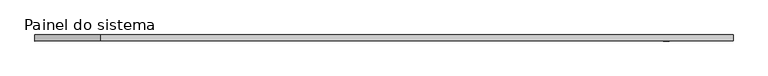
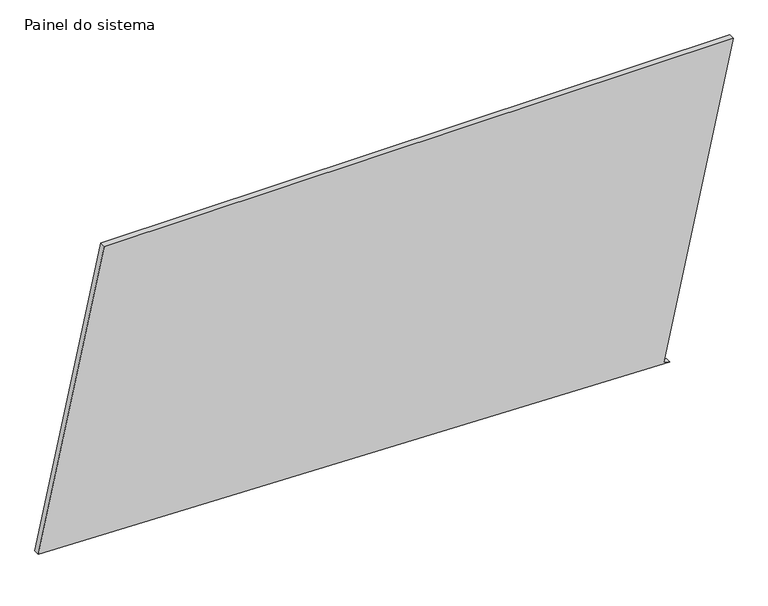
"""IFC4 building model written with IfcOpenShell, lengths in millimetres: plate geometry, Painel do sistema : Envidraçado."""

from ifc_helpers import new_model, si_unit, frame, origin, place, context, project, spatial, polyline, outline, extrude, source, transform, mapped, element, save


def painel_do_sistema_9cf679a2(model_context):
    return source(origin(), model_context, "Body", "SweptSolid", [
        extrude(outline(polyline([(0.0, 1177.0888965), (5.3087357, 1152.6590515), (1326.6613714, 1439.7960293), (1326.6613714, -1167.2906666), (72.6407921, -1439.7960293), (0.0, 1177.0888965)])), frame((0.0, 24.5, 0.0), z_axis=(0.0, 1.0, 0.0), x_axis=(0.0, 0.0, 1.0)), (0.0, 0.0, 1.0), 25.0),
    ])


if __name__ == "__main__":
    model = new_model("IFC4")
    model_context = context("Model", 3, world=origin())
    ifc_project = project(units=[si_unit("LENGTHUNIT", "METRE", prefix="MILLI")], contexts=[model_context])
    site = spatial("IfcSite", under=ifc_project)
    building = spatial("IfcBuilding", under=site)
    placement = place(None, origin())
    painel_do_sistema_shape = painel_do_sistema_9cf679a2(model_context)
    element("IfcPlate", 1, ObjectType="Painel do sistema : Envidraçado", at=placement, inside=building, context=model_context, shape_type="MappedRepresentation", body=[
        mapped(painel_do_sistema_shape, transform((0.0, 0.0, 0.0), x_axis=(1.0, 0.0, 0.0), y_axis=(0.0, 1.0, 0.0), z_axis=(0.0, 0.0, 1.0))),
    ])
    save(model, "model.ifc")

# Revit data of these elements
# Type "Painel do sistema : Envidraçado"
#   Construction Type Id = "GSP4R"
#   Analytic Construction = "Vidraça única Pilkington 1/8 pol"
#   Visual Light Transmittance = 0.9
#   Solar Heat Gain Coefficient = 0.86
#   Heat Transfer Coefficient (U) = 6.7069 W/(m²·K)
# Element 1 (IfcPlate, "Painel do sistema : Envidraçado")
#   Materials on its faces: "Vidro"
# Materials
#   "Vidro": class "Vidro", colour RGB 0 128 192, transparency 0.9, Description = "Vidro de sílica", Cost = 0
